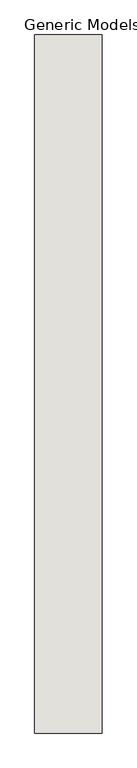
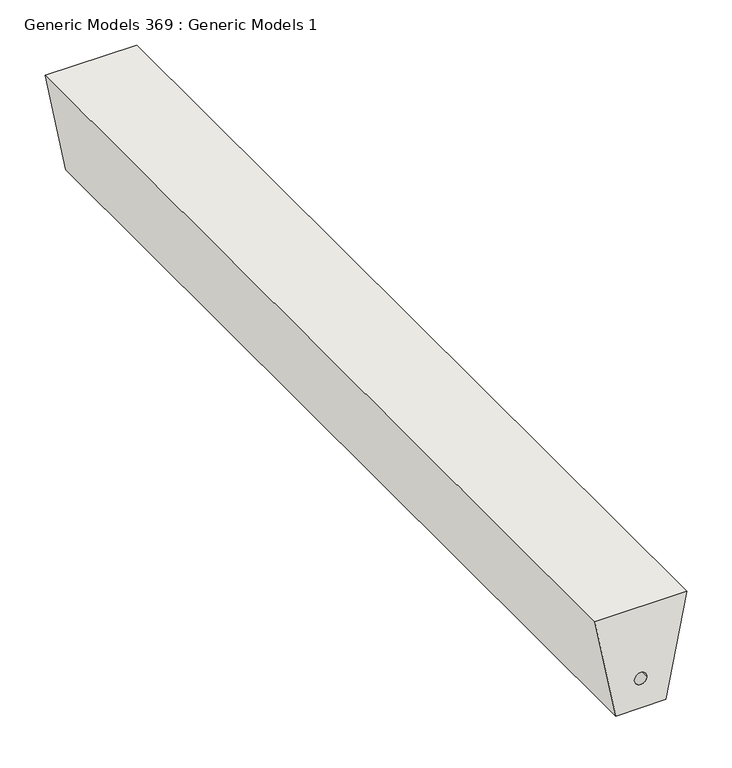
"""IFC4 building model written with IfcOpenShell, lengths in millimetres: wall geometry, Generic Models 369 : Generic Models 1."""

from ifc_helpers import new_model, si_unit, point, frame, frame_2d, origin, place, context, project, spatial, polyline, circle_curve, trimmed, segment, composite_curve, outline, extrude, source, transform, mapped, element, save


def generic_models_369_generic_models_1_a6e56821(model_context):
    return source(origin(), model_context, "Body", "SweptSolid", [
        extrude(outline(polyline([(2225.675, 148524.9125), (2225.675, 148407.4375), (2088.5416825, 148434.0935167), (2088.5416825, 148498.2564833), (2225.675, 148524.9125)]), holes=[composite_curve([segment(trimmed(circle_curve(frame_2d((2128.2291825, 148466.175)), 7.9375), [point((2128.2291825, 148458.2375))], [point((2128.2291825, 148474.1125))], True, "CARTESIAN"), True, "CONTINUOUS"), segment(trimmed(circle_curve(frame_2d((2128.2291825, 148466.175)), 7.9375), [point((2128.2291825, 148474.1125))], [point((2128.2291825, 148458.2375))], True, "CARTESIAN"), True, "CONTINUOUS")], self_intersect=False)]), frame((0.0, 0.0, 0.0), z_axis=(0.0, 1.0, 0.0), x_axis=(0.0, 0.0, 1.0)), (0.0, 0.0, 1.0), 1219.2),
    ])


if __name__ == "__main__":
    model = new_model("IFC4")
    model_context = context("Model", 3, world=origin())
    ifc_project = project(units=[si_unit("LENGTHUNIT", "METRE", prefix="MILLI")], contexts=[model_context])
    site = spatial("IfcSite", under=ifc_project)
    building = spatial("IfcBuilding", under=site)
    placement = place(None, origin())
    generic_models_369_generic_models_1_shape = generic_models_369_generic_models_1_a6e56821(model_context)
    element("IfcWall", 1, ObjectType="Generic Models 369 : Generic Models 1", at=placement, inside=building, context=model_context, shape_type="MappedRepresentation", body=[
        mapped(generic_models_369_generic_models_1_shape, transform((0.0, 0.0, 0.0), x_axis=(1.0, 0.0, 0.0), y_axis=(0.0, 1.0, 0.0), z_axis=(0.0, 0.0, 1.0))),
    ])
    save(model, "model.ifc")

# Revit data of these elements
# Element 1 (IfcWall, "Generic Models 369 : Generic Models 1")
#   Materials on its faces: "FILL CORE IF APPLICABLE - SEE STRUCTURAL DWGS FOR DETAILS"
# Materials
#   "FILL CORE IF APPLICABLE - SEE STRUCTURAL DWGS FOR DETAILS": class "Generic", colour RGB 170 170 170, transparency 0, Cost = 0
